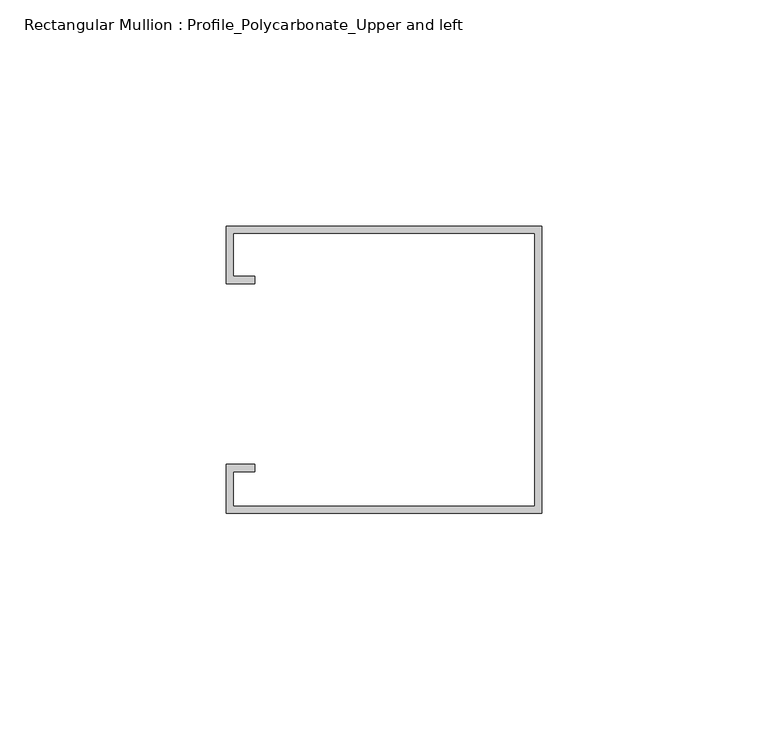
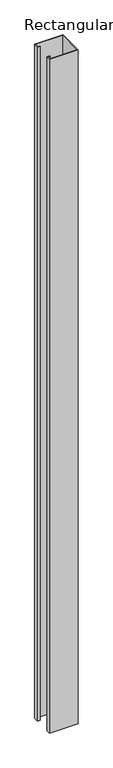
"""IFC4 building model written with IfcOpenShell, lengths in millimetres: member geometry, Rectangular Mullion : Profile_Polycarbonate_Upper and left."""

from ifc_helpers import new_model, si_unit, frame, origin, place, context, project, spatial, polyline, outline, extrude, source, transform, mapped, element, save


def rectangular_mullion_profile_polycarbonate_upper_and_left_9428fc4d(model_context):
    return source(origin(), model_context, "Body", "SweptSolid", [
        extrude(outline(polyline([(0.0, 32.7), (0.0, -30.8), (-69.85, -30.8), (-69.85, -20.0), (-63.5, -20.0), (-63.5, -21.5875), (-68.2625, -21.5875), (-68.2625, -29.2125), (-1.5875, -29.2125), (-1.5875, 31.1125), (-68.2625, 31.1125), (-68.2625, 21.5875), (-63.5, 21.5875), (-63.5, 20.0), (-69.85, 20.0), (-69.85, 32.7), (0.0, 32.7)])), frame((0.0, 0.0, -1752.6), z_axis=(0.0, 0.0, 1.0), x_axis=(1.0, 0.0, 0.0)), (0.0, 0.0, 1.0), 1752.6),
    ])


if __name__ == "__main__":
    model = new_model("IFC4")
    model_context = context("Model", 3, world=origin())
    ifc_project = project(units=[si_unit("LENGTHUNIT", "METRE", prefix="MILLI")], contexts=[model_context])
    site = spatial("IfcSite", under=ifc_project)
    building = spatial("IfcBuilding", under=site)
    placement = place(None, origin())
    rectangular_mullion_profile_polycarbonate_upper_and_left_shape = rectangular_mullion_profile_polycarbonate_upper_and_left_9428fc4d(model_context)
    element("IfcMember", 1, ObjectType="Rectangular Mullion : Profile_Polycarbonate_Upper and left", at=placement, inside=building, context=model_context, shape_type="MappedRepresentation", body=[
        mapped(rectangular_mullion_profile_polycarbonate_upper_and_left_shape, transform((0.0, 0.0, 0.0), x_axis=(1.0, 0.0, 0.0), y_axis=(0.0, 1.0, 0.0), z_axis=(0.0, 0.0, 1.0))),
    ])
    save(model, "model.ifc")

# Revit data of these elements
# Type "Rectangular Mullion : Profile_Polycarbonate_Upper and left"
#   built-in parameter 1007322 = 0.208333 (stored number, unit not read)
#   built-in parameter 1007321 = 0.00520833 (stored number, unit not read)
#   built-in parameter 1007320 = 0 (stored number, unit not read)
# Element 1 (IfcMember, "Rectangular Mullion : Profile_Polycarbonate_Upper and left")
#   Materials on its faces: "GALVANIZED UNISTRUT P5500, 1 5/8\" X 2 7/16\" OR ALUM. CHANNEL"
# Materials
#   "GALVANIZED UNISTRUT P5500, 1 5/8\" X 2 7/16\" OR ALUM. CHANNEL": class "Metal", colour RGB 244 244 244, transparency 0, Description = "Aluminum 6061", Cost = 0
